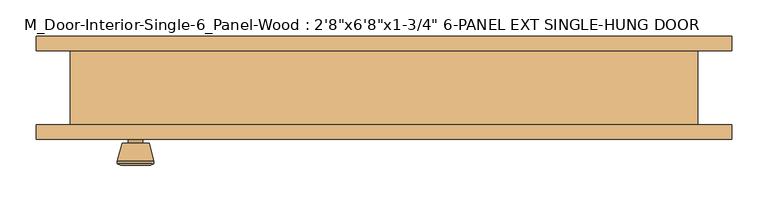
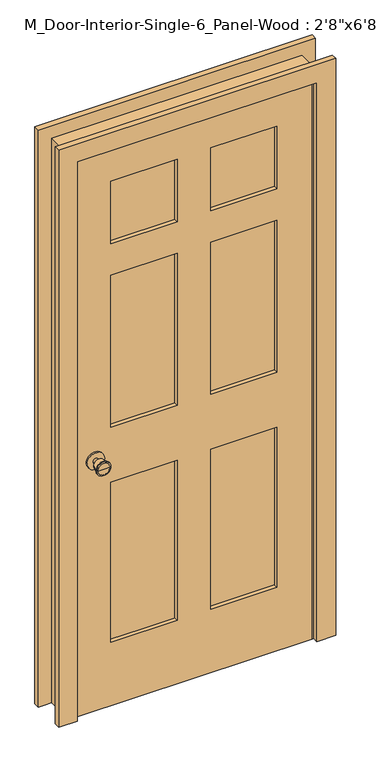
"""IFC4 building model written with IfcOpenShell, lengths in millimetres: door geometry."""

from ifc_helpers import new_model, si_unit, point, frame, frame_2d, origin, place, context, project, spatial, polyline, circle_curve, trimmed, segment, composite_curve, outline, extrude, faceted_brep, source, transform, mapped, element, save
from ifc_brep_helpers import plane_surface, cylinder_surface, revolved_surface, advanced_brep


def door_73e27cd9(model_context):
    return source(origin(), model_context, "Body", "SolidModel", [
        advanced_brep(
        [(-341.4, 2.825, 914.4), (-351.4, 2.825, 914.4), (-331.4, 2.825, 914.4), (-320.9241324, 51.825, 914.4), (-361.8758676, 51.825, 914.4), (-341.4, 51.825, 914.4), (-316.4, 49.9971319, 914.4), (-366.4, 49.9971319, 914.4), (-316.4, 46.5334537, 914.4), (-366.4, 46.5334537, 914.4), (-322.763764, 21.825, 914.4), (-360.036236, 21.825, 914.4), (-331.4, 21.825, 914.4), (-351.4, 21.825, 914.4)],
        [
            (0, 1),
            (1, 2, circle_curve(frame((-341.4, 2.825, 914.4), z_axis=(0.0, -1.0, 0.0), x_axis=(-1.0, 0.0, 0.0)), 10.0)),
            (2, 0),
            (2, 1, circle_curve(frame((-341.4, 2.825, 914.4), z_axis=(0.0, -1.0, 0.0), x_axis=(-1.0, 0.0, 0.0)), 10.0)),
            (3, 4, circle_curve(frame((-341.4, 51.825, 914.4), z_axis=(0.0, 1.0, 0.0), x_axis=(-1.0, 0.0, 0.0)), 20.4758676)),
            (4, 5),
            (5, 3),
            (4, 3, circle_curve(frame((-341.4, 51.825, 914.4), z_axis=(0.0, 1.0, 0.0), x_axis=(-1.0, 0.0, 0.0)), 20.4758676)),
            (6, 7, circle_curve(frame((-341.4, 49.9971319, 914.4), z_axis=(0.0, 1.0, 0.0), x_axis=(-1.0, 0.0, 0.0)), 25.0)),
            (7, 4),
            (3, 6),
            (7, 6, circle_curve(frame((-341.4, 49.9971319, 914.4), z_axis=(0.0, 1.0, 0.0), x_axis=(-1.0, 0.0, 0.0)), 25.0)),
            (8, 9, circle_curve(frame((-341.4, 46.5334537, 914.4), z_axis=(0.0, 1.0, 0.0), x_axis=(-1.0, 0.0, 0.0)), 25.0)),
            (9, 7),
            (6, 8),
            (9, 8, circle_curve(frame((-341.4, 46.5334537, 914.4), z_axis=(0.0, 1.0, 0.0), x_axis=(-1.0, 0.0, 0.0)), 25.0)),
            (10, 11, circle_curve(frame((-341.4, 21.825, 914.4), z_axis=(0.0, 1.0, 0.0), x_axis=(-1.0, 0.0, 0.0)), 18.636236)),
            (11, 9),
            (8, 10),
            (11, 10, circle_curve(frame((-341.4, 21.825, 914.4), z_axis=(0.0, 1.0, 0.0), x_axis=(-1.0, 0.0, 0.0)), 18.636236)),
            (12, 13, circle_curve(frame((-341.4, 21.825, 914.4), z_axis=(0.0, 1.0, 0.0), x_axis=(-1.0, 0.0, 0.0)), 10.0)),
            (13, 11),
            (10, 12),
            (13, 12, circle_curve(frame((-341.4, 21.825, 914.4), z_axis=(0.0, 1.0, 0.0), x_axis=(-1.0, 0.0, 0.0)), 10.0)),
            (1, 13),
            (12, 2),
        ],
        [
            plane_surface(frame((-341.4, 2.825, 914.4), z_axis=(0.0, -1.0, 0.0), x_axis=(-1.0, 0.0, 0.0))),
            plane_surface(frame((-341.4, 51.825, 914.4), z_axis=(0.0, 1.0, 0.0), x_axis=(-1.0, 0.0, 0.0))),
            revolved_surface(polyline([(-361.8758676, 51.825, 914.4), (-366.4, 49.9971319, 914.4)]), (-341.4, 2.825, 914.4), (0.0, -1.0, 0.0)),
            cylinder_surface(frame((-341.4, 2.825, 914.4), z_axis=(0.0, -1.0, 0.0), x_axis=(-1.0, 0.0, 0.0)), 25.0),
            revolved_surface(polyline([(-366.4, 46.5334537, 914.4), (-360.036236, 21.825, 914.4)]), (-341.4, 2.825, 914.4), (0.0, -1.0, 0.0)),
            plane_surface(frame((-341.4, 21.825, 914.4), z_axis=(0.0, -1.0, 0.0), x_axis=(-1.0, 0.0, 0.0))),
            cylinder_surface(frame((-341.4, 2.825, 914.4), z_axis=(0.0, -1.0, 0.0), x_axis=(-1.0, 0.0, 0.0)), 10.0),
        ],
        [
            (0, [[1, 2, 3]]),
            (0, [[-3, 4, -1]]),
            (1, [[5, 6, 7]]),
            (1, [[8, -7, -6]]),
            (2, [[9, 10, -5, 11]]),
            (2, [[12, -11, -8, -10]]),
            (3, [[13, 14, -9, 15]]),
            (3, [[16, -15, -12, -14]]),
            (4, [[17, 18, -13, 19]]),
            (4, [[20, -19, -16, -18]]),
            (5, [[21, 22, -17, 23]]),
            (5, [[24, -23, -20, -22]]),
            (6, [[-2, 25, -21, 26]]),
            (6, [[-4, -26, -24, -25]]),
        ],
    ),
        extrude(outline(composite_curve([segment(trimmed(circle_curve(frame_2d((914.4, -341.4)), 30.0), [point((914.4, -371.4))], [point((914.4, -311.4))], False, "CARTESIAN"), True, "CONTINUOUS"), segment(trimmed(circle_curve(frame_2d((914.4, -341.4)), 30.0), [point((914.4, -311.4))], [point((914.4, -371.4))], False, "CARTESIAN"), True, "CONTINUOUS")], self_intersect=False)), frame((0.0, -3.175, 0.0), z_axis=(0.0, 1.0, 0.0), x_axis=(0.0, 0.0, 1.0)), (0.0, 0.0, 1.0), 6.0),
        advanced_brep(
        [(-341.4, -53.625, 914.4), (-331.4, -53.625, 914.4), (-351.4, -53.625, 914.4), (-320.9241324, -102.625, 914.4), (-341.4, -102.625, 914.4), (-361.8758676, -102.625, 914.4), (-316.4, -100.7971319, 914.4), (-366.4, -100.7971319, 914.4), (-316.4, -97.3334537, 914.4), (-366.4, -97.3334537, 914.4), (-322.763764, -72.625, 914.4), (-360.036236, -72.625, 914.4), (-331.4, -72.625, 914.4), (-351.4, -72.625, 914.4)],
        [
            (0, 1),
            (1, 2, circle_curve(frame((-341.4, -53.625, 914.4), z_axis=(0.0, 1.0, 0.0), x_axis=(-1.0, 0.0, 0.0)), 10.0)),
            (2, 0),
            (2, 1, circle_curve(frame((-341.4, -53.625, 914.4), z_axis=(0.0, 1.0, 0.0), x_axis=(-1.0, 0.0, 0.0)), 10.0)),
            (3, 4),
            (4, 5),
            (5, 3, circle_curve(frame((-341.4, -102.625, 914.4), z_axis=(0.0, -1.0, 0.0), x_axis=(-1.0, 0.0, 0.0)), 20.4758676)),
            (3, 5, circle_curve(frame((-341.4, -102.625, 914.4), z_axis=(0.0, -1.0, 0.0), x_axis=(-1.0, 0.0, 0.0)), 20.4758676)),
            (6, 3),
            (5, 7),
            (7, 6, circle_curve(frame((-341.4, -100.7971319, 914.4), z_axis=(0.0, -1.0, 0.0), x_axis=(-1.0, 0.0, 0.0)), 25.0)),
            (6, 7, circle_curve(frame((-341.4, -100.7971319, 914.4), z_axis=(0.0, -1.0, 0.0), x_axis=(-1.0, 0.0, 0.0)), 25.0)),
            (8, 6),
            (7, 9),
            (9, 8, circle_curve(frame((-341.4, -97.3334537, 914.4), z_axis=(0.0, -1.0, 0.0), x_axis=(-1.0, 0.0, 0.0)), 25.0)),
            (8, 9, circle_curve(frame((-341.4, -97.3334537, 914.4), z_axis=(0.0, -1.0, 0.0), x_axis=(-1.0, 0.0, 0.0)), 25.0)),
            (10, 8),
            (9, 11),
            (11, 10, circle_curve(frame((-341.4, -72.625, 914.4), z_axis=(0.0, -1.0, 0.0), x_axis=(-1.0, 0.0, 0.0)), 18.636236)),
            (10, 11, circle_curve(frame((-341.4, -72.625, 914.4), z_axis=(0.0, -1.0, 0.0), x_axis=(-1.0, 0.0, 0.0)), 18.636236)),
            (12, 10),
            (11, 13),
            (13, 12, circle_curve(frame((-341.4, -72.625, 914.4), z_axis=(0.0, -1.0, 0.0), x_axis=(-1.0, 0.0, 0.0)), 10.0)),
            (12, 13, circle_curve(frame((-341.4, -72.625, 914.4), z_axis=(0.0, -1.0, 0.0), x_axis=(-1.0, 0.0, 0.0)), 10.0)),
            (1, 12),
            (13, 2),
        ],
        [
            plane_surface(frame((-341.4, -53.625, 914.4), z_axis=(0.0, 1.0, 0.0), x_axis=(-1.0, 0.0, 0.0))),
            plane_surface(frame((-341.4, -102.625, 914.4), z_axis=(0.0, -1.0, 0.0), x_axis=(-1.0, 0.0, 0.0))),
            revolved_surface(polyline([(-361.8758676, -102.625, 914.4), (-366.4, -100.7971319, 914.4)]), (-341.4, -53.625, 914.4), (0.0, 1.0, 0.0)),
            cylinder_surface(frame((-341.4, -53.625, 914.4), z_axis=(0.0, 1.0, 0.0), x_axis=(-1.0, 0.0, 0.0)), 25.0),
            revolved_surface(polyline([(-366.4, -97.3334537, 914.4), (-360.036236, -72.625, 914.4)]), (-341.4, -53.625, 914.4), (0.0, 1.0, 0.0)),
            plane_surface(frame((-341.4, -72.625, 914.4), z_axis=(0.0, 1.0, 0.0), x_axis=(-1.0, 0.0, 0.0))),
            cylinder_surface(frame((-341.4, -53.625, 914.4), z_axis=(0.0, 1.0, 0.0), x_axis=(-1.0, 0.0, 0.0)), 10.0),
        ],
        [
            (0, [[1, 2, 3]]),
            (0, [[-3, 4, -1]]),
            (1, [[5, 6, 7]]),
            (1, [[-6, -5, 8]]),
            (2, [[9, -7, 10, 11]]),
            (2, [[-10, -8, -9, 12]]),
            (3, [[13, -11, 14, 15]]),
            (3, [[-14, -12, -13, 16]]),
            (4, [[17, -15, 18, 19]]),
            (4, [[-18, -16, -17, 20]]),
            (5, [[21, -19, 22, 23]]),
            (5, [[-22, -20, -21, 24]]),
            (6, [[25, -23, 26, -2]]),
            (6, [[-26, -24, -25, -4]]),
        ],
    ),
        extrude(outline(composite_curve([segment(trimmed(circle_curve(frame_2d((914.4, -341.4)), 30.0), [point((914.4, -371.4))], [point((914.4, -311.4))], False, "CARTESIAN"), True, "CONTINUOUS"), segment(trimmed(circle_curve(frame_2d((914.4, -341.4)), 30.0), [point((914.4, -311.4))], [point((914.4, -371.4))], False, "CARTESIAN"), True, "CONTINUOUS")], self_intersect=False)), frame((0.0, -53.625, 0.0), z_axis=(0.0, 1.0, 0.0), x_axis=(0.0, 0.0, 1.0)), (0.0, 0.0, 1.0), 6.0),
        extrude(outline(polyline([(286.4, -17.9916667), (286.4, -32.8083333), (57.5, -32.8083333), (57.5, -17.9916667), (286.4, -17.9916667)])), frame((0.0, 0.0, 1683.1), z_axis=(0.0, 0.0, 1.0), x_axis=(1.0, 0.0, 0.0)), (0.0, 0.0, 1.0), 228.9),
        extrude(outline(polyline([(286.4, -17.9916667), (286.4, -32.8083333), (57.5, -32.8083333), (57.5, -17.9916667), (286.4, -17.9916667)])), frame((0.0, 0.0, 1014.4), z_axis=(0.0, 0.0, 1.0), x_axis=(1.0, 0.0, 0.0)), (0.0, 0.0, 1.0), 553.7),
        extrude(outline(polyline([(-57.5, -17.9916667), (-57.5, -32.8083333), (-286.4, -32.8083333), (-286.4, -17.9916667), (-57.5, -17.9916667)])), frame((0.0, 0.0, 1014.4), z_axis=(0.0, 0.0, 1.0), x_axis=(1.0, 0.0, 0.0)), (0.0, 0.0, 1.0), 553.7),
        extrude(outline(polyline([(-57.5, -17.9916667), (-57.5, -32.8083333), (-286.4, -32.8083333), (-286.4, -17.9916667), (-57.5, -17.9916667)])), frame((0.0, 0.0, 1683.1), z_axis=(0.0, 0.0, 1.0), x_axis=(1.0, 0.0, 0.0)), (0.0, 0.0, 1.0), 228.9),
        extrude(outline(polyline([(286.4, -17.9916667), (286.4, -32.8083333), (57.5, -32.8083333), (57.5, -17.9916667), (286.4, -17.9916667)])), frame((0.0, 0.0, 230.0), z_axis=(0.0, 0.0, 1.0), x_axis=(1.0, 0.0, 0.0)), (0.0, 0.0, 1.0), 584.4),
        extrude(outline(polyline([(-57.5, -17.9916667), (-57.5, -32.8083333), (-286.4, -32.8083333), (-286.4, -17.9916667), (-57.5, -17.9916667)])), frame((0.0, 0.0, 230.0), z_axis=(0.0, 0.0, 1.0), x_axis=(1.0, 0.0, 0.0)), (0.0, 0.0, 1.0), 584.4),
        extrude(outline(polyline([(2032.0, -406.4), (0.0, -406.4), (0.0, 406.4), (2032.0, 406.4), (2032.0, -406.4)]), holes=[polyline([(1912.0, 57.5), (1912.0, 286.4), (1683.1, 286.4), (1683.1, 57.5), (1912.0, 57.5)]), polyline([(1568.1, 286.4), (1014.4, 286.4), (1014.4, 57.5), (1568.1, 57.5), (1568.1, 286.4)]), polyline([(1014.4, -57.5), (1014.4, -286.4), (1568.1, -286.4), (1568.1, -57.5), (1014.4, -57.5)]), polyline([(1683.1, -286.4), (1912.0, -286.4), (1912.0, -57.5), (1683.1, -57.5), (1683.1, -286.4)]), polyline([(814.4, 57.5), (814.4, 286.4), (230.0, 286.4), (230.0, 57.5), (814.4, 57.5)]), polyline([(230.0, -57.5), (230.0, -286.4), (814.4, -286.4), (814.4, -57.5), (230.0, -57.5)])]), frame((0.0, -47.625, 0.0), z_axis=(0.0, 1.0, 0.0), x_axis=(0.0, 0.0, 1.0)), (0.0, 0.0, 1.0), 44.45),
        faceted_brep([(431.4, -47.625, 0.0), (406.4, -47.625, 0.0), (406.4, -3.175, 0.0), (393.7, -3.175, 0.0), (393.7, 31.75, 0.0), (406.4, 31.75, 0.0), (406.4, 53.975, 0.0), (431.4, 53.975, 0.0), (431.4, 53.975, 2057.0), (431.4, -47.625, 2057.0), (406.4, 53.975, 2032.0), (-406.4, 53.975, 2032.0), (-406.4, 53.975, 0.0), (-431.4, 53.975, 0.0), (-431.4, 53.975, 2057.0), (406.4, 31.75, 2032.0), (393.7, 31.75, 2019.3), (-393.7, 31.75, 2019.3), (-393.7, 31.75, 0.0), (-406.4, 31.75, 0.0), (-406.4, 31.75, 2032.0), (393.7, -3.175, 2019.3), (406.4, -3.175, 2032.0), (-406.4, -3.175, 2032.0), (-406.4, -3.175, 0.0), (-393.7, -3.175, 0.0), (-393.7, -3.175, 2019.3), (406.4, -47.625, 2032.0), (-431.4, -47.625, 2057.0), (-431.4, -47.625, 0.0), (-406.4, -47.625, 0.0), (-406.4, -47.625, 2032.0)], [[[0, 1, 2, 3, 4, 5, 6, 7]], [[7, 8, 9, 0]], [[6, 10, 11, 12, 13, 14, 8, 7]], [[5, 15, 10, 6]], [[4, 16, 17, 18, 19, 20, 15, 5]], [[3, 21, 16, 4]], [[2, 22, 23, 24, 25, 26, 21, 3]], [[1, 27, 22, 2]], [[0, 9, 28, 29, 30, 31, 27, 1]], [[8, 14, 28, 9]], [[15, 20, 11, 10]], [[21, 26, 17, 16]], [[27, 31, 23, 22]], [[29, 13, 12, 19, 18, 25, 24, 30]], [[14, 13, 29, 28]], [[20, 19, 12, 11]], [[26, 25, 18, 17]], [[31, 30, 24, 23]]]),
        extrude(outline(polyline([(0.0, 477.75), (2103.35, 477.75), (2103.35, -477.75), (0.0, -477.75), (0.0, -412.75), (2038.35, -412.75), (2038.35, 412.75), (0.0, 412.75), (0.0, 477.75)])), frame((0.0, 53.975, 0.0), z_axis=(0.0, 1.0, 0.0), x_axis=(0.0, 0.0, 1.0)), (0.0, 0.0, 1.0), 20.0),
        extrude(outline(polyline([(0.0, 477.75), (2103.35, 477.75), (2103.35, -477.75), (0.0, -477.75), (0.0, -412.75), (2038.35, -412.75), (2038.35, 412.75), (0.0, 412.75), (0.0, 477.75)])), frame((0.0, -67.625, 0.0), z_axis=(0.0, 1.0, 0.0), x_axis=(0.0, 0.0, 1.0)), (0.0, 0.0, 1.0), 20.0),
    ])


if __name__ == "__main__":
    model = new_model("IFC4")
    model_context = context("Model", 3, world=origin())
    ifc_project = project(units=[si_unit("LENGTHUNIT", "METRE", prefix="MILLI")], contexts=[model_context])
    site = spatial("IfcSite", under=ifc_project)
    building = spatial("IfcBuilding", under=site)
    placement = place(None, origin())
    door_shape = door_73e27cd9(model_context)
    element("IfcDoor", 1, ObjectType="M_Door-Interior-Single-6_Panel-Wood : 2'8\"x6'8\"x1-3/4\" 6-PANEL EXT SINGLE-HUNG DOOR", at=placement, inside=building, context=model_context, shape_type="MappedRepresentation", body=[
        mapped(door_shape, transform((0.0, 0.0, 0.0), x_axis=(1.0, 0.0, 0.0), y_axis=(0.0, 1.0, 0.0), z_axis=(0.0, 0.0, 1.0))),
    ])
    save(model, "model.ifc")

# Revit data of these elements
# Type "M_Door-Interior-Single-6_Panel-Wood : 2'8\"x6'8\"x1-3/4\" 6-PANEL EXT SINGLE-HUNG DOOR"
#   Type Mark = "37"
#   Assembly Code = "C1020300"
#   Analytic Construction = "Wooden"
#   Top Rail = 0' - 4.72441"
#   Top Panel = 0' - 9.01181"
#   Thickness = 0' - 1 3/4"
#   Thermal Resistance (R) = 2.5876 (h·ft²·°F)/BTU
#   Swing Angle [instance default] = 90.00°
#   Stiles = 0' - 4.72441"
#   Rough Width = 2' - 9.9685"
#   Rough Height = 6' - 8.98425"
#   Mullion = 0' - 4.52756"
#   Lock Rail = 0' - 7.87402"
#   Intermediate Rail = 0' - 4.52756"
#   Height = 6' - 8"
#   Width = 2' - 8"
#   Heat Transfer Coefficient (U) = 0.3865 BTU/(h·ft²·°F)
#   Bottom Rail = 0' - 9.05512"
#   Trim Material = Cherry
#   Panel Material = Cherry
#   Frame Material = Cherry
#   Door Handle Material = Aluminum
#   Visual Light Transmittance = 0
#   Solar Heat Gain Coefficient = 0
#   Wall Closure = (empty or 0)
#   Function = (empty or 0)
# Element 1 (IfcDoor, "M_Door-Interior-Single-6_Panel-Wood : 2'8\"x6'8\"x1-3/4\" 6-PANEL EXT SINGLE-HUNG DOOR")
#   Materials on its faces: "Cherry", "Aluminum"
# Materials
#   "Cherry": class "Wood", colour RGB 226 177 128, transparency 0, Description = "Prunus Serotina", Cost = 0
#   "Aluminum": class "Metal", colour RGB 244 244 244, transparency 0, Description = "Aluminum 6061", Cost = 0
